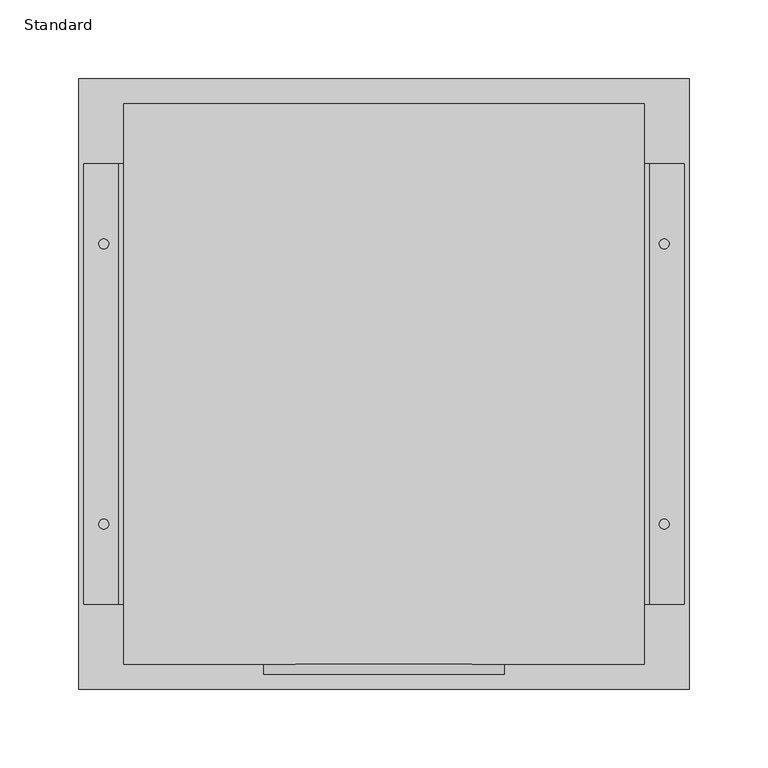
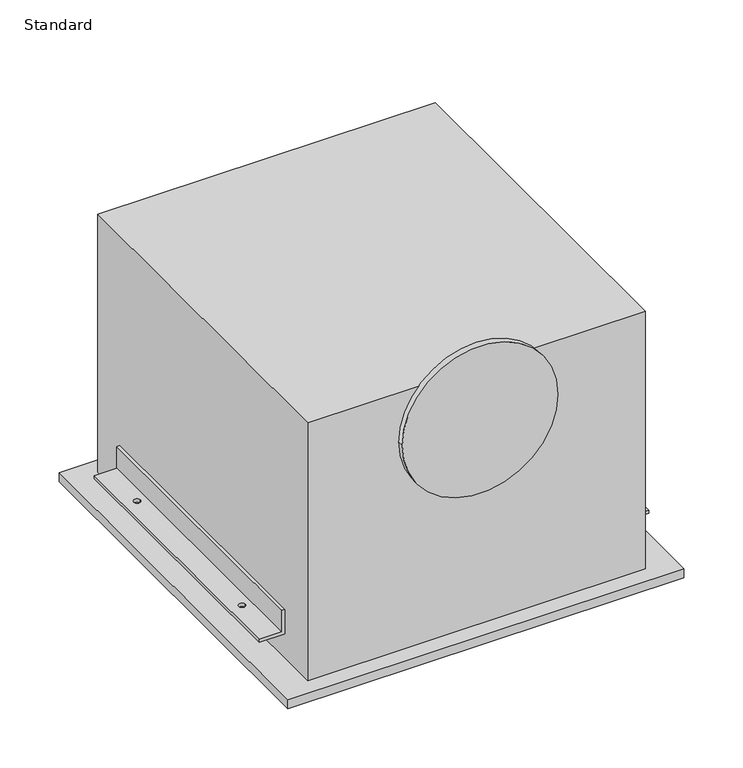
"""IFC4 building model written with IfcOpenShell, lengths in millimetres: proxy geometry, Ceiling-Exhaust-SP-A : Standard."""

from ifc_helpers import new_model, si_unit, point, frame, frame_2d, origin, origin_with_axes, place, context, project, spatial, polyline, circle_curve, trimmed, segment, composite_curve, outline, extrude, source, transform, mapped, element, save
from ifc_brep_helpers import plane_surface, revolved_surface, advanced_brep


def standard_97cd8053(model_context):
    return source(origin(), model_context, "Body", "SolidModel", [
        extrude(outline(polyline([(101.6, 193.0115232), (101.6, -162.5884768), (-228.6, -162.5884768), (-228.6, 193.0115232), (101.6, 193.0115232)])), origin_with_axes(), (0.0, 0.0, 1.0), 266.7),
        extrude(outline(polyline([(130.175, -178.4634768), (-257.175, -178.4634768), (-257.175, 208.8865232), (130.175, 208.8865232), (130.175, -178.4634768)])), frame((0.0, 0.0, -9.525), z_axis=(0.0, 0.0, 1.0), x_axis=(1.0, 0.0, 0.0)), (0.0, 0.0, 1.0), 9.525),
        extrude(outline(composite_curve([segment(trimmed(circle_curve(frame_2d((215.9, -63.5)), 76.2), [point((215.9, -139.7))], [point((215.9, 12.7))], False, "CARTESIAN"), True, "CONTINUOUS"), segment(trimmed(circle_curve(frame_2d((215.9, -63.5)), 76.2), [point((215.9, 12.7))], [point((215.9, -139.7))], False, "CARTESIAN"), True, "CONTINUOUS")], self_intersect=False)), frame((0.0, -168.9384768, 0.0), z_axis=(0.0, 1.0, 0.0), x_axis=(0.0, 0.0, 1.0)), (0.0, 0.0, 1.0), 6.35),
        advanced_brep(
        [(127.0, -124.4884768, 25.4), (127.0, -124.4884768, 28.575), (104.775, -124.4884768, 28.575), (104.775, -124.4884768, 50.8), (101.6, -124.4884768, 50.8), (101.6, -124.4884768, 25.4), (127.0, 154.9115232, 25.4), (101.6, 154.9115232, 25.4), (101.6, 154.9115232, 50.8), (104.775, 154.9115232, 50.8), (104.775, 154.9115232, 28.575), (127.0, 154.9115232, 28.575), (117.475, -73.6884768, 28.575), (111.125, -73.6884768, 28.575), (117.475, 104.1115232, 28.575), (111.125, 104.1115232, 28.575), (111.125, -73.6884768, 25.4), (117.475, -73.6884768, 25.4), (111.125, 104.1115232, 25.4), (117.475, 104.1115232, 25.4)],
        [
            (0, 1),
            (1, 2),
            (2, 3),
            (3, 4),
            (4, 5),
            (5, 0),
            (6, 7),
            (7, 8),
            (8, 9),
            (9, 10),
            (10, 11),
            (11, 6),
            (0, 6),
            (11, 1),
            (10, 2),
            (12, 13, circle_curve(frame((114.3, -73.6884768, 28.575), z_axis=(0.0, 0.0, -1.0), x_axis=(1.0, 0.0, 0.0)), 3.175)),
            (13, 12, circle_curve(frame((114.3, -73.6884768, 28.575), z_axis=(0.0, 0.0, -1.0), x_axis=(1.0, 0.0, 0.0)), 3.175)),
            (14, 15, circle_curve(frame((114.3, 104.1115232, 28.575), z_axis=(0.0, 0.0, -1.0), x_axis=(1.0, 0.0, 0.0)), 3.175)),
            (15, 14, circle_curve(frame((114.3, 104.1115232, 28.575), z_axis=(0.0, 0.0, -1.0), x_axis=(1.0, 0.0, 0.0)), 3.175)),
            (9, 3),
            (8, 4),
            (7, 5),
            (16, 17, circle_curve(frame((114.3, -73.6884768, 25.4), z_axis=(0.0, 0.0, 1.0), x_axis=(1.0, 0.0, 0.0)), 3.175)),
            (17, 16, circle_curve(frame((114.3, -73.6884768, 25.4), z_axis=(0.0, 0.0, 1.0), x_axis=(1.0, 0.0, 0.0)), 3.175)),
            (18, 19, circle_curve(frame((114.3, 104.1115232, 25.4), z_axis=(0.0, 0.0, 1.0), x_axis=(1.0, 0.0, 0.0)), 3.175)),
            (19, 18, circle_curve(frame((114.3, 104.1115232, 25.4), z_axis=(0.0, 0.0, 1.0), x_axis=(1.0, 0.0, 0.0)), 3.175)),
            (12, 17),
            (16, 13),
            (14, 19),
            (18, 15),
        ],
        [
            plane_surface(frame((127.0, -124.4884768, 25.4), z_axis=(0.0, -1.0, 0.0), x_axis=(0.0, 0.0, 1.0))),
            plane_surface(frame((127.0, 154.9115232, 25.4), z_axis=(0.0, 1.0, 0.0), x_axis=(0.0, 0.0, -1.0))),
            plane_surface(frame((127.0, -124.4884768, 25.4), z_axis=(1.0, 0.0, 0.0), x_axis=(0.0, 1.0, 0.0))),
            plane_surface(frame((127.0, -124.4884768, 28.575), z_axis=(0.0, 0.0, 1.0), x_axis=(0.0, 1.0, 0.0))),
            plane_surface(frame((104.775, -124.4884768, 28.575), z_axis=(1.0, 0.0, 0.0), x_axis=(0.0, 1.0, 0.0))),
            plane_surface(frame((104.775, -124.4884768, 50.8), z_axis=(0.0, 0.0, 1.0), x_axis=(0.0, 1.0, 0.0))),
            plane_surface(frame((101.6, -124.4884768, 50.8), z_axis=(-1.0, 0.0, 0.0), x_axis=(0.0, 1.0, 0.0))),
            plane_surface(frame((101.6, -124.4884768, 25.4), z_axis=(0.0, 0.0, -1.0), x_axis=(0.0, 1.0, 0.0))),
            revolved_surface(polyline([(117.475, -73.6884768, 28.575), (117.475, -73.6884768, 25.4)]), (114.3, -73.6884768, 0.0), (0.0, 0.0, 1.0)),
            revolved_surface(polyline([(117.475, 104.1115232, 28.575), (117.475, 104.1115232, 25.4)]), (114.3, 104.1115232, 0.0), (0.0, 0.0, 1.0)),
        ],
        [
            (0, [[1, 2, 3, 4, 5, 6]]),
            (1, [[7, 8, 9, 10, 11, 12]]),
            (2, [[-1, 13, -12, 14]]),
            (3, [[-2, -14, -11, 15], [16, 17], [18, 19]]),
            (4, [[-3, -15, -10, 20]]),
            (5, [[-4, -20, -9, 21]]),
            (6, [[-5, -21, -8, 22]]),
            (7, [[-6, -22, -7, -13], [23, 24], [25, 26]]),
            (8, [[27, -23, 28, -16]]),
            (8, [[-27, -17, -28, -24]]),
            (9, [[29, -25, 30, -18]]),
            (9, [[-29, -19, -30, -26]]),
        ],
    ),
        advanced_brep(
        [(-254.0, -124.4884768, 25.4), (-228.6, -124.4884768, 25.4), (-228.6, -124.4884768, 50.8), (-231.775, -124.4884768, 50.8), (-231.775, -124.4884768, 28.575), (-254.0, -124.4884768, 28.575), (-254.0, 154.9115232, 25.4), (-254.0, 154.9115232, 28.575), (-231.775, 154.9115232, 28.575), (-231.775, 154.9115232, 50.8), (-228.6, 154.9115232, 50.8), (-228.6, 154.9115232, 25.4), (-244.475, 104.1115232, 25.4), (-238.125, 104.1115232, 25.4), (-244.475, -73.6884768, 25.4), (-238.125, -73.6884768, 25.4), (-238.125, 104.1115232, 28.575), (-244.475, 104.1115232, 28.575), (-238.125, -73.6884768, 28.575), (-244.475, -73.6884768, 28.575)],
        [
            (0, 1),
            (1, 2),
            (2, 3),
            (3, 4),
            (4, 5),
            (5, 0),
            (6, 7),
            (7, 8),
            (8, 9),
            (9, 10),
            (10, 11),
            (11, 6),
            (0, 6),
            (11, 1),
            (12, 13, circle_curve(frame((-241.3, 104.1115232, 25.4), z_axis=(0.0, 0.0, 1.0), x_axis=(1.0, 0.0, 0.0)), 3.175)),
            (13, 12, circle_curve(frame((-241.3, 104.1115232, 25.4), z_axis=(0.0, 0.0, 1.0), x_axis=(1.0, 0.0, 0.0)), 3.175)),
            (14, 15, circle_curve(frame((-241.3, -73.6884768, 25.4), z_axis=(0.0, 0.0, 1.0), x_axis=(1.0, 0.0, 0.0)), 3.175)),
            (15, 14, circle_curve(frame((-241.3, -73.6884768, 25.4), z_axis=(0.0, 0.0, 1.0), x_axis=(1.0, 0.0, 0.0)), 3.175)),
            (10, 2),
            (9, 3),
            (8, 4),
            (7, 5),
            (16, 17, circle_curve(frame((-241.3, 104.1115232, 28.575), z_axis=(0.0, 0.0, -1.0), x_axis=(1.0, 0.0, 0.0)), 3.175)),
            (17, 16, circle_curve(frame((-241.3, 104.1115232, 28.575), z_axis=(0.0, 0.0, -1.0), x_axis=(1.0, 0.0, 0.0)), 3.175)),
            (18, 19, circle_curve(frame((-241.3, -73.6884768, 28.575), z_axis=(0.0, 0.0, -1.0), x_axis=(1.0, 0.0, 0.0)), 3.175)),
            (19, 18, circle_curve(frame((-241.3, -73.6884768, 28.575), z_axis=(0.0, 0.0, -1.0), x_axis=(1.0, 0.0, 0.0)), 3.175)),
            (16, 13),
            (12, 17),
            (18, 15),
            (14, 19),
        ],
        [
            plane_surface(frame((-228.6, -124.4884768, 25.4), z_axis=(0.0, -1.0, 0.0), x_axis=(1.0, 0.0, 0.0))),
            plane_surface(frame((-228.6, 154.9115232, 25.4), z_axis=(0.0, 1.0, 0.0), x_axis=(-1.0, 0.0, 0.0))),
            plane_surface(frame((-254.0, -124.4884768, 25.4), z_axis=(0.0, 0.0, -1.0), x_axis=(0.0, 1.0, 0.0))),
            plane_surface(frame((-228.6, -124.4884768, 25.4), z_axis=(1.0, 0.0, 0.0), x_axis=(0.0, 1.0, 0.0))),
            plane_surface(frame((-228.6, -124.4884768, 50.8), z_axis=(0.0, 0.0, 1.0), x_axis=(0.0, 1.0, 0.0))),
            plane_surface(frame((-231.775, -124.4884768, 50.8), z_axis=(-1.0, 0.0, 0.0), x_axis=(0.0, 1.0, 0.0))),
            plane_surface(frame((-231.775, -124.4884768, 28.575), z_axis=(0.0, 0.0, 1.0), x_axis=(0.0, 1.0, 0.0))),
            plane_surface(frame((-254.0, -124.4884768, 28.575), z_axis=(-1.0, 0.0, 0.0), x_axis=(0.0, 1.0, 0.0))),
            revolved_surface(polyline([(-238.125, 104.1115232, 28.575), (-238.125, 104.1115232, 25.4)]), (-241.3, 104.1115232, 25.4), (0.0, 0.0, 1.0)),
            revolved_surface(polyline([(-238.125, -73.6884768, 28.575), (-238.125, -73.6884768, 25.4)]), (-241.3, -73.6884768, 0.0), (0.0, 0.0, 1.0)),
        ],
        [
            (0, [[1, 2, 3, 4, 5, 6]]),
            (1, [[7, 8, 9, 10, 11, 12]]),
            (2, [[-1, 13, -12, 14], [15, 16], [17, 18]]),
            (3, [[-2, -14, -11, 19]]),
            (4, [[-3, -19, -10, 20]]),
            (5, [[-4, -20, -9, 21]]),
            (6, [[-5, -21, -8, 22], [23, 24], [25, 26]]),
            (7, [[-6, -22, -7, -13]]),
            (8, [[27, -15, 28, -23]]),
            (8, [[-27, -24, -28, -16]]),
            (9, [[29, -17, 30, -25]]),
            (9, [[-29, -26, -30, -18]]),
        ],
    ),
    ])


if __name__ == "__main__":
    model = new_model("IFC4")
    model_context = context("Model", 3, world=origin())
    ifc_project = project(units=[si_unit("LENGTHUNIT", "METRE", prefix="MILLI")], contexts=[model_context])
    site = spatial("IfcSite", under=ifc_project)
    building = spatial("IfcBuilding", under=site)
    placement = place(None, origin())
    standard_shape = standard_97cd8053(model_context)
    element("IfcBuildingElementProxy", 1, Name="Ceiling-Exhaust-SP-A : Standard", ObjectType="Ceiling-Exhaust-SP-A : Standard", at=placement, inside=building, context=model_context, shape_type="MappedRepresentation", body=[
        mapped(standard_shape, transform((0.0, 0.0, 0.0), x_axis=(1.0, 0.0, 0.0), y_axis=(0.0, 1.0, 0.0), z_axis=(0.0, 0.0, 1.0))),
    ])
    save(model, "model.ifc")

# Revit data of these elements
# Type "Ceiling-Exhaust-SP-A : Standard"
#   Type Mark = "Ceiling-Exhaust-SP-A"
#   COBie.Type.CreatedBy = "info@mma.ie"
#   COBie.Type.CreatedOn = "2017-07-21T10:57:54"
#   COBie.Type.Name = "Ceiling-Exhaust-SP-A"
#   COBie.Type.Category = "23-33 41 17 11 : Constant Volume Air Terminal Units"
#   COBie.Type.Description = "Ceiling-Exhaust-SP-A_Standard"
#   COBie.Type.AssetType = "Fixed"
#   COBie.Type.Manufacturer = ""
#   COBie.Type.ModelNumber = ""
#   COBie.Type.ModelReference = ""
#   Classification.OmniClass.21.Number = "21-04 30 60 30"
#   Classification.OmniClass.21.Description = "Exhaust Air"
#   Classification.OmniClass.23.Number = "23-33 41 17 11"
#   Classification.OmniClass.23.Description = "Constant Volume Air Terminal Units"
#   Version Family = "rfa 1.0"
#   Version Data = "NA"
#   Keynote = "23 35 00.A"
#   Copyright © = ""
#   COBie.Type.ReplacementCost = 0
#   Voltage [instance default] = 0 V
#   Static Pressure = 0.0 in-wg
#   Sones = 3.5 CFM
#   Round Duct Offset [instance default] = 50.8 mm
#   Mounting Width = 177.8 mm
#   Mounting Length = 355.6 mm
#   Half Mounting Width = 88.9 mm
#   Grille Width = 387.35 mm
#   Grille Length = 387.35 mm
#   Grille Height = 266.7 mm
#   Grill Width = 355.6 mm
#   Grill Lenght = 330.2 mm
#   Frequency = 60 Hz
#   Electrical Load [instance default] = 0 VA
#   Duct Width = 152.4 mm
#   Duct Radius [instance default] = 76.2 mm
#   Duct Height = 152.4 mm
#   Ceiling Radiation Damper Height [instance default] = 0 mm
#   Base Width = 355.6 mm
#   Base Length = 330.2 mm
#   Base Height = 266.7 mm
#   Air Volume [instance default] = 70.0 CFM
#   Air Flow = 100.0 CFM
#   COBie.Type = yes
#   VFD [instance default] = no
#   Round Connection Selection [instance default] = yes
#   Rectangular Connection Selection [instance default] = no
#   Number of Poles [instance default] = 1
#   Ceiling Radiation Damper Selection [instance default] = no
#   URL = ""
#   Model = ""
#   Manufacturer = ""
#   Description = (empty or 0)
#   Default Elevation = 0
#   Assembly Code = ""
# Element 1 (IfcBuildingElementProxy, "Ceiling-Exhaust-SP-A : Standard")
#   Voltage = 230 V
#   Materials on its faces: "Default"
# Materials
#   "Default": class "Miscellaneous", colour RGB 127 127 127, transparency 0
